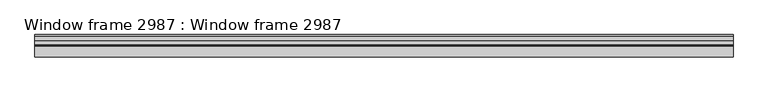
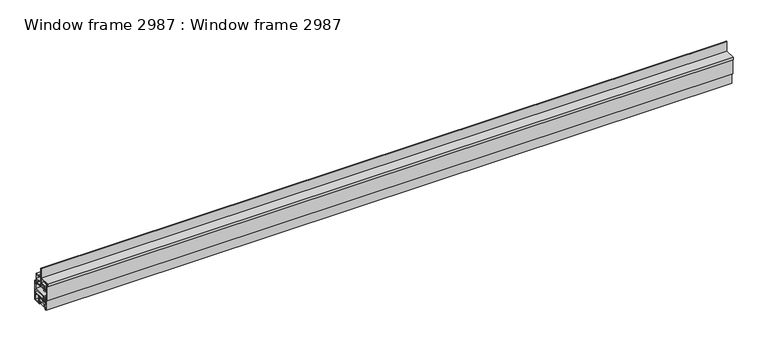
"""IFC4 building model written with IfcOpenShell, lengths in millimetres: proxy geometry, Window frame 2987 : Window frame 2987."""

from ifc_helpers import new_model, si_unit, frame, origin, place, context, project, spatial, polyline, outline, extrude, source, transform, mapped, element, save


def window_frame_2987_window_frame_2987_9ad6bbad(model_context):
    return source(origin(), model_context, "Body", "SweptSolid", [
        extrude(outline(polyline([(10418.5923445, 42826.6453557), (10419.7664569, 42826.6453557), (10420.4289839, 42824.0551381), (10420.4289839, 42822.1937752), (10419.7933448, 42819.331799), (10418.4399798, 42819.331799), (10418.0162385, 42821.7906919), (10415.7900245, 42821.7906919), (10415.7900245, 42824.2036919), (10418.0169323, 42824.2036919), (10418.5923445, 42826.6453557)])), frame((3694.2883192, 0.0, 0.0), z_axis=(1.0, 0.0, 0.0), x_axis=(0.0, 1.0, 0.0)), (0.0, 0.0, 1.0), 2000.0),
        extrude(outline(polyline([(10448.2175044, 42819.8677418), (10447.0433921, 42819.8677418), (10446.3808651, 42822.4579594), (10446.3808651, 42824.3193223), (10447.0165042, 42827.1812985), (10448.3698692, 42827.1812985), (10448.7936105, 42824.7224056), (10451.0198245, 42824.7224056), (10451.0198245, 42822.3094056), (10448.7929166, 42822.3094056), (10448.2175044, 42819.8677418)])), frame((3694.2883192, 0.0, 0.0), z_axis=(1.0, 0.0, 0.0), x_axis=(0.0, 1.0, 0.0)), (0.0, 0.0, 1.0), 2000.0),
        extrude(outline(polyline([(10465.1041245, 42877.4063057), (10465.9357049, 42877.4063057), (10465.9357049, 42874.4580592), (10469.2316245, 42874.4580592), (10469.2316245, 42873.2642592), (10465.9357049, 42873.2642592), (10465.9357049, 42869.8889235), (10465.1041245, 42869.8889235), (10465.1041245, 42877.4063057)])), frame((3694.2883192, 0.0, 0.0), z_axis=(1.0, 0.0, 0.0), x_axis=(0.0, 1.0, 0.0)), (0.0, 0.0, 1.0), 2000.0),
        extrude(outline(polyline([(10413.9358245, 42853.8568749), (10413.1042441, 42853.8568749), (10413.1042441, 42856.8051214), (10409.8083245, 42856.8051214), (10409.8083245, 42857.9989214), (10413.1042441, 42857.9989214), (10413.1042441, 42861.374257), (10413.9358245, 42861.374257), (10413.9358245, 42853.8568749)])), frame((3694.2883192, 0.0, 0.0), z_axis=(1.0, 0.0, 0.0), x_axis=(0.0, 1.0, 0.0)), (0.0, 0.0, 1.0), 2000.0),
        extrude(outline(polyline([(10418.4443245, 42902.8807214), (10418.4443245, 42900.8487214), (10409.9861245, 42900.8487214), (10409.9861245, 42889.6981214), (10413.7961245, 42889.6981214), (10413.7961245, 42885.6014104), (10412.3731145, 42885.6014104), (10412.3731145, 42887.6214119), (10409.9861245, 42887.6214119), (10409.9861245, 42878.1157214), (10412.3737249, 42878.1157214), (10412.3737249, 42879.920664), (10413.7961245, 42879.920664), (10413.7961245, 42878.1157214), (10415.4227819, 42878.1157214), (10415.4227819, 42876.0837214), (10412.3483245, 42876.0837214), (10412.3483245, 42859.2695099), (10411.087306, 42859.2695099), (10411.087306, 42860.1579214), (10409.8083245, 42860.1579214), (10409.8083245, 42855.0779214), (10411.0783245, 42855.0779214), (10411.0783245, 42856.0691163), (10412.3483245, 42856.0691163), (10412.3483245, 42853.8079214), (10407.9541245, 42853.8079214), (10407.9541245, 42902.8807214), (10418.4443245, 42902.8807214)])), frame((3694.2883192, 0.0, 0.0), z_axis=(1.0, 0.0, 0.0), x_axis=(0.0, 1.0, 0.0)), (0.0, 0.0, 1.0), 2000.0),
        extrude(outline(polyline([(10428.4773245, 42839.9141214), (10430.6490245, 42839.9141214), (10430.6490245, 42838.5425214), (10427.0764417, 42838.5425214), (10427.0764417, 42841.7175214), (10425.348612, 42841.7175214), (10425.348612, 42843.7495178), (10429.9378245, 42843.7495178), (10429.9378245, 42853.2999214), (10427.3814153, 42853.2999214), (10427.3814153, 42852.0547043), (10426.1278245, 42852.0547043), (10426.1278245, 42855.3319214), (10466.6916245, 42855.3319214), (10466.6916245, 42872.1780411), (10467.9847912, 42872.1780411), (10467.9847912, 42871.2711655), (10469.2316245, 42871.2711655), (10469.2316245, 42876.3349778), (10467.9855642, 42876.3349778), (10467.9855642, 42875.3379685), (10466.6916245, 42875.3379685), (10466.6916245, 42877.6077214), (10471.0858245, 42877.6077214), (10471.0858245, 42836.8915214), (10467.6363003, 42836.8915214), (10469.0538245, 42839.6863677), (10469.0538245, 42841.7175214), (10428.4773245, 42841.7175214), (10428.4773245, 42839.9141214)]), holes=[polyline([(10468.5458245, 42852.1569214), (10431.9698245, 42852.1569214), (10431.9698245, 42844.8925214), (10468.5458245, 42844.8925214), (10468.5458245, 42852.1569214)])]), frame((3694.2883192, 0.0, 0.0), z_axis=(1.0, 0.0, 0.0), x_axis=(0.0, 1.0, 0.0)), (0.0, 0.0, 1.0), 2000.0),
        extrude(outline(polyline([(10421.78887, 42832.1417214), (10420.02357, 42833.6676129), (10420.02357, 42838.4388847), (10418.3300245, 42838.4388847), (10418.3300245, 42841.7175214), (10425.1480856, 42841.7175214), (10425.1480856, 42838.0201392), (10432.0614644, 42838.0201392), (10432.0614644, 42839.8688303), (10446.1049245, 42839.8887214), (10446.1049245, 42832.1417214), (10421.78887, 42832.1417214)])), frame((3694.2883192, 0.0, 0.0), z_axis=(1.0, 0.0, 0.0), x_axis=(0.0, 1.0, 0.0)), (0.0, 0.0, 1.0), 2000.0),
        extrude(outline(polyline([(3694.2883192, 10427.0041245), (3694.2883192, 10439.7803245), (5694.2883192, 10439.7803245), (5694.2883192, 10427.0041245), (3694.2883192, 10427.0041245)])), frame((0.0, 0.0, 42822.6167214), z_axis=(0.0, 0.0, 1.0), x_axis=(1.0, 0.0, 0.0)), (0.0, 0.0, 1.0), 9.525),
        extrude(outline(polyline([(10415.9678245, 42855.3319214), (10419.7565488, 42855.3319214), (10419.7565488, 42852.0410935), (10418.5352773, 42852.0410935), (10418.5352773, 42853.2999214), (10415.9678245, 42853.2999214), (10415.9678245, 42843.7495178), (10420.5652242, 42843.7495178), (10420.5652242, 42841.7175214), (10418.3300245, 42841.7175214), (10418.3300245, 42824.9283463), (10417.0702123, 42824.9283463), (10417.0702123, 42825.7917214), (10415.7900245, 42825.7917214), (10415.7900245, 42820.7117214), (10417.0878667, 42820.7117214), (10417.0878667, 42821.695665), (10418.3300245, 42821.695665), (10418.3300245, 42819.4417214), (10413.9358245, 42819.4417214), (10413.9358245, 42860.1579214), (10415.9678245, 42860.1579214), (10415.9678245, 42855.3319214)])), frame((3694.2883192, 0.0, 0.0), z_axis=(1.0, 0.0, 0.0), x_axis=(0.0, 1.0, 0.0)), (0.0, 0.0, 1.0), 2000.0),
        extrude(outline(polyline([(10421.4124692, 42887.6661214), (10421.4124692, 42885.6014104), (10420.1461245, 42885.6014104), (10420.1461245, 42889.6981214), (10439.7041254, 42889.6981217), (10439.7041245, 42902.9006541), (10439.7041245, 42933.2282541), (10441.2789245, 42933.2282541), (10441.2789245, 42889.6981214), (10463.0721245, 42889.6981214), (10463.0721245, 42900.8487214), (10454.6139245, 42900.8487214), (10454.6139245, 42902.8807214), (10465.1041245, 42902.8807214), (10465.1041245, 42871.2577214), (10461.6954078, 42871.2577214), (10463.0721245, 42873.8234791), (10463.0721245, 42876.0837214), (10422.4174665, 42876.0837214), (10422.4174665, 42874.2803214), (10425.3549991, 42874.2803214), (10425.3549991, 42872.9087214), (10421.1188154, 42872.9087214), (10421.1188154, 42876.0837214), (10419.3669123, 42876.0837214), (10419.3669123, 42878.1157214), (10423.9561245, 42878.1157214), (10423.9561245, 42887.6661214), (10421.4124692, 42887.6661214)]), holes=[polyline([(10432.9456415, 42879.2587214), (10432.9456415, 42878.1157214), (10441.2754602, 42878.1157214), (10441.2754602, 42879.2587214), (10445.1719198, 42879.2587214), (10445.1719198, 42878.1157214), (10449.6566572, 42878.1157214), (10449.6566572, 42879.2587214), (10458.5370268, 42879.2587214), (10458.5370268, 42878.1157214), (10462.5641245, 42878.1157214), (10462.5641245, 42887.6661214), (10458.5827674, 42887.6661214), (10458.5827674, 42886.5231214), (10454.6623354, 42886.5231214), (10454.6623354, 42887.6661214), (10445.0988588, 42887.6661214), (10445.0988588, 42886.5231214), (10439.3964147, 42886.5231214), (10439.3964147, 42887.6661214), (10429.6250371, 42887.6661214), (10429.6250371, 42886.5231214), (10425.9881245, 42886.5231214), (10425.9881245, 42879.2587214), (10432.9456415, 42879.2587214)])]), frame((3694.2883192, 0.0, 0.0), z_axis=(1.0, 0.0, 0.0), x_axis=(0.0, 1.0, 0.0)), (0.0, 0.0, 1.0), 2000.0),
        extrude(outline(polyline([(10471.0858245, 42819.4417214), (10448.4674367, 42819.4417214), (10448.4674367, 42821.6504838), (10449.706254, 42821.6504838), (10449.706254, 42820.7213761), (10451.0198245, 42820.7213761), (10451.0198245, 42825.7917214), (10449.6736545, 42825.7917214), (10449.6736545, 42824.8942276), (10448.5000391, 42824.8942276), (10448.5000391, 42827.0778443), (10451.0198245, 42827.0778443), (10451.0198245, 42839.8887214), (10428.4773245, 42839.9141214), (10428.4773245, 42841.2857214), (10452.4168245, 42841.2857214), (10452.4168245, 42820.8387214), (10469.6888245, 42820.8387214), (10469.6888245, 42835.4945214), (10466.2631111, 42835.4945214), (10466.2631111, 42840.581308), (10467.0692386, 42840.581308), (10468.5642504, 42839.1350647), (10467.5710156, 42836.8915214), (10471.0858245, 42836.8915214), (10471.0858245, 42819.4417214)])), frame((3694.2883192, 0.0, 0.0), z_axis=(1.0, 0.0, 0.0), x_axis=(0.0, 1.0, 0.0)), (0.0, 0.0, 1.0), 2000.0),
        extrude(outline(polyline([(10439.7041245, 42934.6307214), (10439.7041245, 42902.8807214), (10407.9541245, 42902.8807214), (10407.9541245, 42896.5307214), (10406.9381245, 42896.5307214), (10406.9381245, 42903.8967214), (10438.6881245, 42903.8967214), (10438.6881245, 42934.6307214), (10439.7041245, 42934.6307214)])), frame((3694.2883192, 0.0, 0.0), z_axis=(1.0, 0.0, 0.0), x_axis=(0.0, 1.0, 0.0)), (0.0, 0.0, 1.0), 2000.0),
    ])


if __name__ == "__main__":
    model = new_model("IFC4")
    model_context = context("Model", 3, world=origin())
    ifc_project = project(units=[si_unit("LENGTHUNIT", "METRE", prefix="MILLI")], contexts=[model_context])
    site = spatial("IfcSite", under=ifc_project)
    building = spatial("IfcBuilding", under=site)
    placement = place(None, origin())
    window_frame_2987_window_frame_2987_shape = window_frame_2987_window_frame_2987_9ad6bbad(model_context)
    element("IfcBuildingElementProxy", 1, Name="Window frame 2987 : Window frame 2987", ObjectType="Window frame 2987 : Window frame 2987", at=placement, inside=building, context=model_context, shape_type="MappedRepresentation", body=[
        mapped(window_frame_2987_window_frame_2987_shape, transform((0.0, 0.0, 0.0), x_axis=(1.0, 0.0, 0.0), y_axis=(0.0, 1.0, 0.0), z_axis=(0.0, 0.0, 1.0))),
    ])
    save(model, "model.ifc")

# Revit data of these elements
# Type "Window frame 2987 : Window frame 2987"
#   NameOverride = "Window frame"
# Element 1 (IfcBuildingElementProxy, "Window frame 2987 : Window frame 2987")
#   Materials on its faces: "FLEETWOOD SERIES 250-T-01 CASEMENT WINDOW FRAME"
# Materials
#   "FLEETWOOD SERIES 250-T-01 CASEMENT WINDOW FRAME": class "Unassigned", colour RGB 128 128 128, transparency 0
